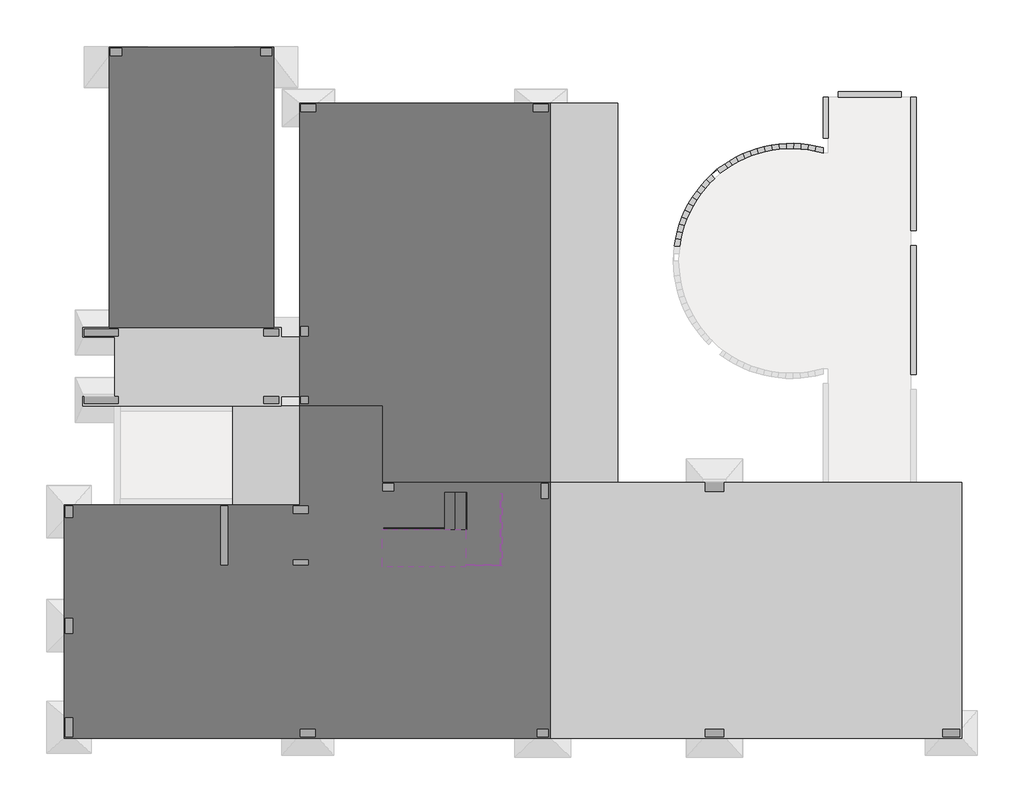
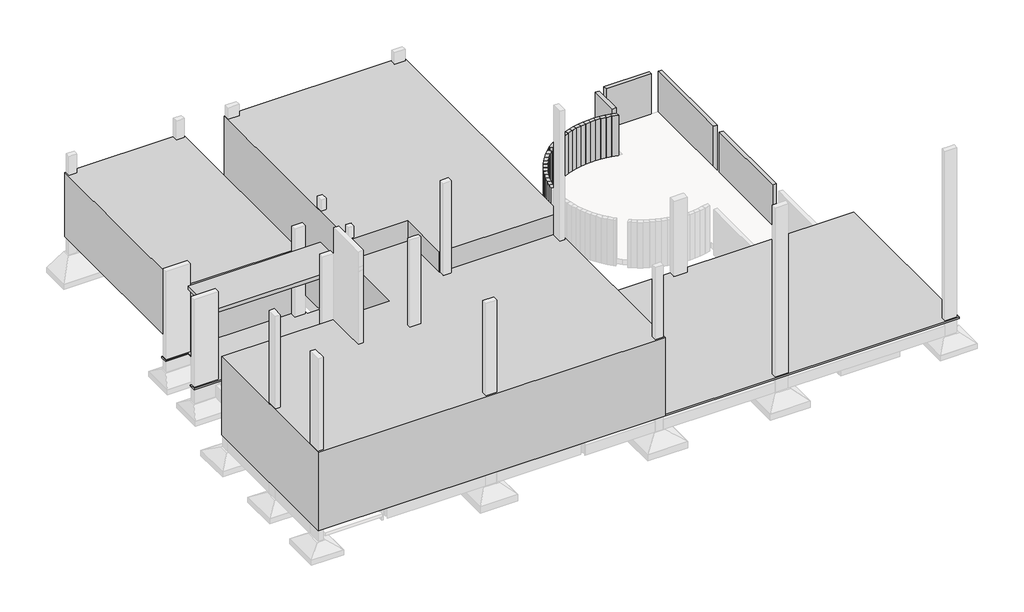
# One storey, part 4 of 4: 29 beams, 7 proxies, 6 railings, 2 stair flights, 1 slab.
"""IFC4 building model written with IfcOpenShell, lengths in millimetres."""

import ifcopenshell
import ifcopenshell.guid

model = None  # the IFC model being written
_history = None  # IfcOwnerHistory: only IFC2X3 demands one
_inside = {}  # id of a spatial element -> (the spatial element, [elements in it])
_under = {}  # id of a project, library or spatial element -> (it, [spatial elements below it])
_declared = {}  # id of a project -> (the project, [libraries it declares])
_typed = {}  # id of a type object -> (the type object, [elements of that type])
_made_of = {}  # id of a material, layer set ... -> (it, [elements and type objects made of it])


def new_model(schema):
    """Start an empty IFC model of exactly this schema.

    Asked for "IFC4X3", IfcOpenShell would pick the latest addendum, in which some entities
    have other attributes; the version numbers below select the first issue.
    IFC2X3 requires an IfcOwnerHistory on every rooted entity: one is made here for all.
    """
    global model, _history
    if schema == "IFC4X3":
        model = ifcopenshell.file(schema_version=(4, 3, 0, 0))
    else:
        model = ifcopenshell.file(schema=schema)
    _inside.clear()
    _under.clear()
    _declared.clear()
    _typed.clear()
    _made_of.clear()
    _history = None
    if model.schema == "IFC2X3":
        org = make("IfcOrganization", Name="unknown")
        user = make(
            "IfcPersonAndOrganization",
            ThePerson=make("IfcPerson", FamilyName="unknown"),
            TheOrganization=org,
        )
        app = make(
            "IfcApplication",
            ApplicationDeveloper=org,
            Version="unknown",
            ApplicationFullName="unknown",
            ApplicationIdentifier="unknown",
        )
        _history = make(
            "IfcOwnerHistory",
            OwningUser=user,
            OwningApplication=app,
            ChangeAction="ADDED",
            CreationDate=0,
        )
    return model


def make(cls, **values):
    """One entity of the class cls with the attributes given. An attribute that is None is left unset."""
    return model.create_entity(
        cls, **{name: value for name, value in values.items() if value is not None}
    )


def rooted(cls, **values):
    """An entity with a GlobalId (a new one), such as an element, a storey or a relation."""
    return make(cls, GlobalId=ifcopenshell.guid.new(), OwnerHistory=_history, **values)


def si_unit(unit_type, name, prefix=None):
    """IfcSIUnit, for example si_unit("LENGTHUNIT", "METRE", prefix="MILLI")."""
    return make("IfcSIUnit", UnitType=unit_type, Prefix=prefix, Name=name)


def assignment(units):
    """IfcUnitAssignment: the units of a project."""
    return None if units is None else make("IfcUnitAssignment", Units=units)


def point(xyz):
    """IfcCartesianPoint."""
    return None if xyz is None else make("IfcCartesianPoint", Coordinates=xyz)


def direction(xyz):
    """IfcDirection."""
    return None if xyz is None else make("IfcDirection", DirectionRatios=xyz)


def frame(location, z_axis=None, x_axis=None):
    """IfcAxis2Placement3D, a coordinate frame: its origin and axes. An axis left out is left unset."""
    return make(
        "IfcAxis2Placement3D",
        Location=point(location),
        Axis=direction(z_axis),
        RefDirection=direction(x_axis),
    )


def origin():
    """The frame at (0, 0, 0) with its axes left unset."""
    return frame((0.0, 0.0, 0.0))


def place(relative_to, where):
    """IfcLocalPlacement: puts the frame where relative to a parent placement (None: the world)."""
    return make(
        "IfcLocalPlacement", PlacementRelTo=relative_to, RelativePlacement=where
    )


def context(
    kind, dimensions, precision=None, world=None, true_north=None, identifier=None
):
    """IfcGeometricRepresentationContext, for example the 3D "Model" context."""
    return make(
        "IfcGeometricRepresentationContext",
        ContextIdentifier=identifier,
        ContextType=kind,
        CoordinateSpaceDimension=dimensions,
        Precision=precision,
        WorldCoordinateSystem=world,
        TrueNorth=true_north,
    )


def project(units=None, contexts=None):
    """IfcProject with its units and contexts."""
    return rooted(
        "IfcProject",
        Name="project",
        RepresentationContexts=contexts,
        UnitsInContext=assignment(units),
    )


def spatial(cls, under=None, at=None, **own):
    """A site, building, storey or space (cls), placed at a placement, below another one or the project."""
    s = rooted(cls, ObjectPlacement=at, **own)
    if under is not None:
        _under.setdefault(under.id(), (under, []))[1].append(s)
    return s


def polyline(points):
    """IfcPolyline through the points."""
    return make("IfcPolyline", Points=[point(p) for p in points])


def outline(outer, holes=None, kind="AREA"):
    """IfcArbitraryClosedProfileDef: a profile drawn as a closed curve; with holes, ...WithVoids."""
    if holes is None:
        return make("IfcArbitraryClosedProfileDef", ProfileType=kind, OuterCurve=outer)
    return make(
        "IfcArbitraryProfileDefWithVoids",
        ProfileType=kind,
        OuterCurve=outer,
        InnerCurves=holes,
    )


def extrude(swept, where, along, depth):
    """IfcExtrudedAreaSolid: the profile swept, set in the frame where, extruded along a direction by depth."""
    return make(
        "IfcExtrudedAreaSolid",
        SweptArea=swept,
        Position=where,
        ExtrudedDirection=direction(along),
        Depth=depth,
    )


def faces_of(points, faces, orient=None, outer=None):
    """IfcFace entities. A face is a list of loops; a loop is a list of indices into points, from 0.

    orient and outer hold one flag for each loop. By default every Orientation is true, the
    first loop of a face is its IfcFaceOuterBound and the others are IfcFaceBound.
    """
    made = []
    for i, loops in enumerate(faces):
        bounds = []
        for j, loop in enumerate(loops):
            is_outer = j == 0 if outer is None else outer[i][j]
            bounds.append(
                make(
                    "IfcFaceOuterBound" if is_outer else "IfcFaceBound",
                    Bound=make("IfcPolyLoop", Polygon=[points[k] for k in loop]),
                    Orientation=True if orient is None else orient[i][j],
                )
            )
        made.append(make("IfcFace", Bounds=bounds))
    return made


def faceted_brep(points, faces, orient=None, outer=None, voids=None):
    """IfcFacetedBrep: a solid bounded by flat faces; with voids (closed shells), ...WithVoids."""
    shared = [point(p) for p in points]
    hull = make("IfcClosedShell", CfsFaces=faces_of(shared, faces, orient, outer))
    if voids is None:
        return make("IfcFacetedBrep", Outer=hull)
    return make(
        "IfcFacetedBrepWithVoids",
        Outer=hull,
        Voids=[
            make(cls, CfsFaces=faces_of(shared, fs, o, b)) for cls, fs, o, b in voids
        ],
    )


def shape(context_of_items, identifier, shape_type, items):
    """IfcShapeRepresentation: the items that make up one representation, for example the "Body"."""
    return make(
        "IfcShapeRepresentation",
        ContextOfItems=context_of_items,
        RepresentationIdentifier=identifier,
        RepresentationType=shape_type,
        Items=items,
    )


def source(mapping_origin, context_of_items, identifier, shape_type, items):
    """IfcRepresentationMap: a shape defined once, which mapped items show again and again."""
    return make(
        "IfcRepresentationMap",
        MappingOrigin=mapping_origin,
        MappedRepresentation=shape(context_of_items, identifier, shape_type, items),
    )


def transform(
    local_origin,
    x_axis=None,
    y_axis=None,
    z_axis=None,
    scale=None,
    scale2=None,
    scale3=None,
    uniform=True,
):
    """IfcCartesianTransformationOperator3D, or its non-uniform kind. x_axis, y_axis, z_axis: its Axis1, 2, 3."""
    if uniform:
        return make(
            "IfcCartesianTransformationOperator3D",
            Axis1=direction(x_axis),
            Axis2=direction(y_axis),
            LocalOrigin=point(local_origin),
            Scale=scale,
            Axis3=direction(z_axis),
        )
    return make(
        "IfcCartesianTransformationOperator3DnonUniform",
        Axis1=direction(x_axis),
        Axis2=direction(y_axis),
        LocalOrigin=point(local_origin),
        Scale=scale,
        Axis3=direction(z_axis),
        Scale2=scale2,
        Scale3=scale3,
    )


def mapped(mapping_source, mapping_target):
    """IfcMappedItem: shows the shape of a source again, moved by a transform."""
    return make(
        "IfcMappedItem", MappingSource=mapping_source, MappingTarget=mapping_target
    )


def made_of(thing, what):
    """Note that an element or type object is made of a material, layer set ...; save() writes the relation."""
    if what is not None:
        _made_of.setdefault(what.id(), (what, []))[1].append(thing)
    return thing


def element(
    cls,
    number,
    at=None,
    inside=None,
    cuts=None,
    type_object=None,
    material=None,
    context=None,
    identifier="Body",
    shape_type=None,
    held_by="IfcProductDefinitionShape",
    body=None,
    shapes=None,
    **own,
):
    """One element of the class cls, such as IfcWall. Its Tag is "e" and its number.

    at: its placement. inside: the storey or other place that contains it. cuts: it is an
    opening in that element (IfcRelVoidsElement). A single representation is given by context,
    identifier, shape_type and body (its items); several are given by shapes. held_by: the class
    of the entity that holds the representations. save() writes the other relations.
    """
    e = rooted(cls, Tag="e%d" % number, ObjectPlacement=at, **own)
    if body is not None:
        shapes = [shape(context, identifier, shape_type, body)]
    if shapes is not None:
        e.Representation = make(held_by, Representations=shapes)
    if inside is not None:
        _inside.setdefault(inside.id(), (inside, []))[1].append(e)
    if cuts is not None:
        rooted(
            "IfcRelVoidsElement", RelatingBuildingElement=cuts, RelatedOpeningElement=e
        )
    if type_object is not None:
        _typed.setdefault(type_object.id(), (type_object, []))[1].append(e)
    return made_of(e, material)


def aggregate(whole, parts):
    """IfcRelAggregates: a whole, such as a stair, and the parts it consists of."""
    return rooted("IfcRelAggregates", RelatingObject=whole, RelatedObjects=parts)


def save(model, path):
    """Write the relations noted so far, then the file.

    IfcRelAggregates (storeys below a building ...), IfcRelContainedInSpatialStructure (elements
    in a storey), IfcRelDefinesByType, IfcRelAssociatesMaterial and IfcRelDeclares: one each for
    every whole, place, type object, material and project.
    """
    for whole, parts in _under.values():
        aggregate(whole, parts)
    for where, things in _inside.values():
        rooted(
            "IfcRelContainedInSpatialStructure",
            RelatedElements=things,
            RelatingStructure=where,
        )
    for kind, things in _typed.values():
        rooted("IfcRelDefinesByType", RelatedObjects=things, RelatingType=kind)
    for what, things in _made_of.values():
        rooted("IfcRelAssociatesMaterial", RelatedObjects=things, RelatingMaterial=what)
    for by, libraries in _declared.values():
        rooted("IfcRelDeclares", RelatingContext=by, RelatedDefinitions=libraries)
    model.write(path)


def railing_81dbcb3b(model_context):
    return source(origin(), model_context, "Body", "SweptSolid", [
        extrude(outline(polyline([(1832.4523952, 3702.0), (1832.4523952, 3594.0), (1856.4523952, 3594.0), (1856.4523952, 3702.0), (1866.9523952, 3702.0), (1866.9523952, 3700.0), (1858.4523952, 3700.0), (1858.4523952, 3592.0), (1830.4523952, 3592.0), (1830.4523952, 3700.0), (1821.9523952, 3700.0), (1821.9523952, 3702.0), (1832.4523952, 3702.0)])), frame((-12226.1487231, 0.0, 0.0), z_axis=(1.0, 0.0, 0.0), x_axis=(0.0, 1.0, 0.0)), (0.0, 0.0, 1.0), 1940.0),
    ])


def railing_0d959ca4(model_context):
    return source(origin(), model_context, "Body", "SweptSolid", [
        extrude(outline(polyline([(-4674.5702584, 2133.3602771), (-4674.5702584, 2121.3602771), (-6610.5702584, 2121.3602771), (-6610.5702584, 2133.3602771), (-4674.5702584, 2133.3602771)])), frame((0.0, 0.0, 4122.0679199), z_axis=(0.0, 0.0, 1.0), x_axis=(1.0, 0.0, 0.0)), (0.0, 0.0, 1.0), 1100.0),
    ])


def railing_24874f95(model_context):
    return source(origin(), model_context, "Body", "SweptSolid", [
        extrude(outline(polyline([(1832.4523952, 3702.0), (1832.4523952, 3594.0), (1856.4523952, 3594.0), (1856.4523952, 3702.0), (1866.9523952, 3702.0), (1866.9523952, 3700.0), (1858.4523952, 3700.0), (1858.4523952, 3592.0), (1830.4523952, 3592.0), (1830.4523952, 3700.0), (1821.9523952, 3700.0), (1821.9523952, 3702.0), (1832.4523952, 3702.0)])), frame((-12226.1487231, 0.0, 0.0), z_axis=(1.0, 0.0, 0.0), x_axis=(0.0, 1.0, 0.0)), (0.0, 0.0, 1.0), 925.0),
    ])


def railing_29f9e2f6(model_context):
    return source(origin(), model_context, "Body", "SweptSolid", [
        extrude(outline(polyline([(-4674.5702584, 2133.3602771), (-4674.5702584, 2121.3602771), (-5595.5702584, 2121.3602771), (-5595.5702584, 2133.3602771), (-4674.5702584, 2133.3602771)])), frame((0.0, 0.0, 4122.0679199), z_axis=(0.0, 0.0, 1.0), x_axis=(1.0, 0.0, 0.0)), (0.0, 0.0, 1.0), 1100.0),
    ])


def railing_c44cfcee(model_context):
    return source(origin(), model_context, "Body", "SweptSolid", [
        extrude(outline(polyline([(1672.2222222, -4460.281307), (500.0, -4460.281307), (1877.7777778, -2220.281307), (3050.0, -2220.281307), (1672.2222222, -4460.281307)])), frame((0.0, -5573.3699847, 0.0), z_axis=(0.0, 1.0, 0.0), x_axis=(0.0, 0.0, 1.0)), (0.0, 0.0, 1.0), 12.0),
    ])


model = new_model("IFC4")

# Units and contexts
model_context = context("Model", 3, world=origin())
ifc_project = project(units=[si_unit("LENGTHUNIT", "METRE", prefix="MILLI")], contexts=[model_context])

# Site, building, storey
site = spatial("IfcSite", under=ifc_project)
building = spatial("IfcBuilding", under=site)
storey = spatial("IfcBuildingStorey", under=building, Name="PAVIMENTO TÉRREO", Elevation=500.0)

# Beams
placement = place(None, origin())
element("IfcBeam", 1, ObjectType="TQS - Viga retangular : 14.0 x 180.0", at=placement, inside=storey, context=model_context, shape_type="SweptSolid", body=[
    extrude(outline(polyline([(9422.718693, 6109.4300153), (9422.718693, 5969.4300153), (7734.718693, 5969.4300153), (7734.718693, 6109.4300153), (9422.718693, 6109.4300153)])), frame((0.0, 0.0, -1450.0), z_axis=(0.0, 0.0, 1.0), x_axis=(1.0, 0.0, 0.0)), (0.0, 0.0, 1.0), 1800.0),
])
element("IfcBeam", 2, ObjectType="TQS - Viga retangular : 14.0 x 180.0", at=placement, inside=storey, context=model_context, shape_type="Brep", body=[
    faceted_brep([(3391.2860591, 2182.1270296, 350.0), (3359.6197005, 1984.821412, 350.0), (3498.5878389, 1967.228978, 350.0), (3528.8128087, 2155.5536418, 350.0), (3498.5878389, 1967.228978, -1250.0), (3498.5878389, 1967.228978, -1450.0), (3528.8128087, 2155.5536418, -1450.0), (3528.8128087, 2155.5536418, -1250.0), (3359.6197005, 1984.821412, -1450.0), (3391.2860591, 2182.1270296, -1450.0)], [[[0, 1, 2, 3]], [[3, 2, 4, 5, 6, 7]], [[6, 5, 8, 9]], [[1, 0, 9, 8]], [[1, 8, 5, 4, 2]], [[0, 3, 7, 6, 9]]]),
])
element("IfcBeam", 3, ObjectType="TQS - Viga retangular : 14.0 x 180.0", at=placement, inside=storey, context=model_context, shape_type="Brep", body=[
    faceted_brep([(3435.4949989, 2377.433408, 350.0), (3391.2860591, 2182.1270296, 350.0), (3528.8128087, 2155.5536418, 350.0), (3571.057344, 2342.1816685, 350.0), (3528.8128087, 2155.5536418, -1250.0), (3528.8128087, 2155.5536418, -1450.0), (3571.057344, 2342.1816685, -1450.0), (3571.057344, 2342.1816685, -1250.0), (3391.2860591, 2182.1270296, -1450.0), (3435.4949989, 2377.433408, -1450.0)], [[[0, 1, 2, 3]], [[3, 2, 4, 5, 6, 7]], [[6, 5, 8, 9]], [[1, 0, 9, 8]], [[1, 8, 5, 4, 2]], [[0, 3, 7, 6, 9]]]),
])
element("IfcBeam", 4, ObjectType="TQS - Viga retangular : 14.0 x 180.0", at=placement, inside=storey, context=model_context, shape_type="Brep", body=[
    faceted_brep([(3491.8466557, 2568.9190116, 350.0), (3435.4949989, 2377.433408, 350.0), (3571.057344, 2342.1816685, 350.0), (3624.8943566, 2525.1223914, 350.0), (3571.057344, 2342.1816685, -1250.0), (3571.057344, 2342.1816685, -1450.0), (3624.8943566, 2525.1223914, -1450.0), (3624.8943566, 2525.1223914, -1250.0), (3435.4949989, 2377.433408, -1450.0), (3491.8466557, 2568.9190116, -1450.0)], [[[0, 1, 2, 3]], [[3, 2, 4, 5, 6, 7]], [[6, 5, 8, 9]], [[1, 0, 9, 8]], [[1, 8, 5, 4, 2]], [[0, 3, 7, 6, 9]]]),
])
element("IfcBeam", 5, ObjectType="TQS - Viga retangular : 14.0 x 180.0", at=placement, inside=storey, context=model_context, shape_type="Brep", body=[
    faceted_brep([(3560.4750252, 2757.0390761, 350.0), (3491.8466557, 2568.9190116, 350.0), (3624.8943566, 2525.1223914, 350.0), (3690.4700641, 2704.8746778, 350.0), (3624.8943566, 2525.1223914, -1250.0), (3624.8943566, 2525.1223914, -1450.0), (3690.4700641, 2704.8746778, -1450.0), (3690.4700641, 2704.8746778, -1250.0), (3491.8466557, 2568.9190116, -1450.0), (3560.4750252, 2757.0390761, -1450.0)], [[[0, 1, 2, 3]], [[3, 2, 4, 5, 6, 7]], [[6, 5, 8, 9]], [[1, 0, 9, 8]], [[1, 8, 5, 4, 2]], [[0, 3, 7, 6, 9]]]),
])
element("IfcBeam", 6, ObjectType="TQS - Viga retangular : 14.0 x 180.0", at=placement, inside=storey, context=model_context, shape_type="Brep", body=[
    faceted_brep([(3640.6668309, 2939.8368394, 350.0), (3560.4750252, 2757.0390761, 350.0), (3690.4700641, 2704.8746778, 350.0), (3767.0835383, 2879.5156103, 350.0), (3690.4700641, 2704.8746778, -1250.0), (3690.4700641, 2704.8746778, -1450.0), (3767.0835383, 2879.5156103, -1450.0), (3767.0835383, 2879.5156103, -1250.0), (3560.4750252, 2757.0390761, -1450.0), (3640.6668309, 2939.8368394, -1450.0)], [[[0, 1, 2, 3]], [[3, 2, 4, 5, 6, 7]], [[6, 5, 8, 9]], [[1, 0, 9, 8]], [[1, 8, 5, 4, 2]], [[0, 3, 7, 6, 9]]]),
])
element("IfcBeam", 7, ObjectType="TQS - Viga retangular : 14.0 x 180.0", at=placement, inside=storey, context=model_context, shape_type="Brep", body=[
    faceted_brep([(3732.4184841, 3117.3686176, 350.0), (3640.6668309, 2939.8368394, 350.0), (3767.0835383, 2879.5156103, 350.0), (3854.7456543, 3049.1344759, 350.0), (3767.0835383, 2879.5156103, -1250.0), (3767.0835383, 2879.5156103, -1450.0), (3854.7456543, 3049.1344759, -1450.0), (3854.7456543, 3049.1344759, -1250.0), (3640.6668309, 2939.8368394, -1450.0), (3732.4184841, 3117.3686176, -1450.0)], [[[0, 1, 2, 3]], [[3, 2, 4, 5, 6, 7]], [[6, 5, 8, 9]], [[1, 0, 9, 8]], [[1, 8, 5, 4, 2]], [[0, 3, 7, 6, 9]]]),
])
element("IfcBeam", 8, ObjectType="TQS - Viga retangular : 14.0 x 180.0", at=placement, inside=storey, context=model_context, shape_type="Brep", body=[
    faceted_brep([(3835.4781404, 3289.0593829, 350.0), (3732.4184841, 3117.3686176, 350.0), (3854.7456543, 3049.1344759, 350.0), (3953.2211063, 3213.1882515, 350.0), (3854.7456543, 3049.1344759, -1250.0), (3854.7456543, 3049.1344759, -1450.0), (3953.2211063, 3213.1882515, -1450.0), (3953.2211063, 3213.1882515, -1250.0), (3732.4184841, 3117.3686176, -1450.0), (3835.4781404, 3289.0593829, -1450.0)], [[[0, 1, 2, 3]], [[3, 2, 4, 5, 6, 7]], [[6, 5, 8, 9]], [[1, 0, 9, 8]], [[1, 8, 5, 4, 2]], [[0, 3, 7, 6, 9]]]),
])
element("IfcBeam", 9, ObjectType="TQS - Viga retangular : 14.0 x 180.0", at=placement, inside=storey, context=model_context, shape_type="Brep", body=[
    faceted_brep([(3949.2418511, 3453.852677, 350.0), (3835.4781404, 3289.0593829, 350.0), (3953.2211063, 3213.1882515, 350.0), (4061.9244879, 3370.6513671, 350.0), (3953.2211063, 3213.1882515, -1250.0), (3953.2211063, 3213.1882515, -1450.0), (4061.9244879, 3370.6513671, -1450.0), (4061.9244879, 3370.6513671, -1250.0), (3835.4781404, 3289.0593829, -1450.0), (3949.2418511, 3453.852677, -1450.0)], [[[0, 1, 2, 3]], [[3, 2, 4, 5, 6, 7]], [[6, 5, 8, 9]], [[1, 0, 9, 8]], [[1, 8, 5, 4, 2]], [[0, 3, 7, 6, 9]]]),
])
element("IfcBeam", 10, ObjectType="TQS - Viga retangular : 14.0 x 180.0", at=placement, inside=storey, context=model_context, shape_type="Brep", body=[
    faceted_brep([(4073.2495799, 3611.0821108, 350.0), (3949.2418511, 3453.852677, 350.0), (4061.9244879, 3370.6513671, 350.0), (4180.416223, 3520.8870709, 350.0), (4061.9244879, 3370.6513671, -1250.0), (4061.9244879, 3370.6513671, -1450.0), (4180.416223, 3520.8870709, -1450.0), (4180.416223, 3520.8870709, -1250.0), (3949.2418511, 3453.852677, -1450.0), (4073.2495799, 3611.0821108, -1450.0)], [[[0, 1, 2, 3]], [[3, 2, 4, 5, 6, 7]], [[6, 5, 8, 9]], [[1, 0, 9, 8]], [[1, 8, 5, 4, 2]], [[0, 3, 7, 6, 9]]]),
])
element("IfcBeam", 11, ObjectType="TQS - Viga retangular : 14.0 x 180.0", at=placement, inside=storey, context=model_context, shape_type="Brep", body=[
    faceted_brep([(4206.9998658, 3760.1118816, 350.0), (4073.2495799, 3611.0821108, 350.0), (4180.416223, 3520.8870709, 350.0), (4308.2171619, 3663.2878479, 350.0), (4180.416223, 3520.8870709, -1250.0), (4180.416223, 3520.8870709, -1450.0), (4308.2171619, 3663.2878479, -1450.0), (4308.2171619, 3663.2878479, -1250.0), (4073.2495799, 3611.0821108, -1450.0), (4206.9998658, 3760.1118816, -1450.0)], [[[0, 1, 2, 3]], [[3, 2, 4, 5, 6, 7]], [[6, 5, 8, 9]], [[1, 0, 9, 8]], [[1, 8, 5, 4, 2]], [[0, 3, 7, 6, 9]]]),
])
element("IfcBeam", 12, ObjectType="TQS - Viga retangular : 14.0 x 180.0", at=placement, inside=storey, context=model_context, shape_type="Brep", body=[
    faceted_brep([(4505.0858129, 4030.990239, 350.0), (4495.3853819, 4043.0011294, 350.0), (4357.8172159, 3908.0548411, 350.0), (4500.8039544, 4027.7001668, 350.0), (4495.3853819, 4043.0011294, -1450.0), (4505.0858129, 4030.990239, -1450.0), (4500.8039544, 4027.7001668, -1450.0), (4357.8172159, 3908.0548411, -1450.0)], [[[0, 1, 2, 3]], [[4, 5, 6, 7]], [[1, 4, 7, 2]], [[4, 1, 0, 5]], [[3, 6, 5, 0]], [[6, 3, 2, 7]]]),
    faceted_brep([(4433.7325967, 3786.411115, 350.0), (4308.2171619, 3663.2878479, 350.0), (4308.2171619, 3663.2878479, -1250.0), (4308.2171619, 3663.2878479, -1450.0), (4433.7325967, 3786.411115, -1450.0), (4433.7325967, 3786.411115, -1250.0), (4346.9865149, 3897.4305598, 350.0), (4346.9865149, 3897.4305598, -1450.0), (4206.9998658, 3760.1118816, 350.0), (4206.9998658, 3760.1118816, -1450.0)], [[[0, 1, 2, 3, 4, 5]], [[6, 0, 5, 4, 7]], [[8, 9, 3, 2, 1]], [[1, 0, 6, 8]], [[4, 3, 9, 7]], [[6, 7, 9, 8]]]),
])
element("IfcBeam", 13, ObjectType="TQS - Viga retangular : 14.0 x 180.0", at=placement, inside=storey, context=model_context, shape_type="Brep", body=[
    faceted_brep([(4707.2476524, 4182.7114576, 350.0), (4495.3853819, 4043.0011294, 350.0), (4505.0858129, 4030.990239, 350.0), (4583.7591724, 3933.5783713, 350.0), (4784.4362281, 4065.9127281, 350.0), (4583.7591724, 3933.5783713, -1450.0), (4742.6545701, 4038.3602567, -1450.0), (4784.4362281, 4065.9127281, -1450.0), (4784.4362281, 4065.9127281, -1250.0), (4495.3853819, 4043.0011294, -1450.0), (4707.2476524, 4182.7114576, -1450.0), (4505.0858129, 4030.990239, -1450.0)], [[[0, 1, 2, 3, 4]], [[4, 3, 5, 6, 7, 8]], [[9, 10, 7, 6, 5, 11]], [[1, 0, 10, 9]], [[1, 9, 11, 5, 3, 2]], [[0, 4, 8, 7, 10]]]),
])
element("IfcBeam", 14, ObjectType="TQS - Viga retangular : 14.0 x 180.0", at=placement, inside=storey, context=model_context, shape_type="Brep", body=[
    faceted_brep([(4828.0654459, 4262.728967, 350.0), (4707.2476524, 4182.7114576, 350.0), (4784.4362281, 4065.9127281, 350.0), (4901.6570883, 4143.547992, 350.0), (4784.4362281, 4065.9127281, -1250.0), (4784.4362281, 4065.9127281, -1450.0), (4901.6570883, 4143.547992, -1450.0), (4901.6570883, 4143.547992, -1250.0), (4707.2476524, 4182.7114576, -1450.0), (4828.0654459, 4262.728967, -1450.0)], [[[0, 1, 2, 3]], [[3, 2, 4, 5, 6, 7]], [[6, 5, 8, 9]], [[1, 0, 9, 8]], [[1, 8, 5, 4, 2]], [[0, 3, 7, 6, 9]]]),
])
element("IfcBeam", 15, ObjectType="TQS - Viga retangular : 14.0 x 180.0", at=placement, inside=storey, context=model_context, shape_type="Brep", body=[
    faceted_brep([(5001.7073563, 4362.4661134, 350.0), (4828.0654459, 4262.728967, 350.0), (4901.6570883, 4143.547992, 350.0), (5067.5752245, 4238.8487257, 350.0), (4901.6570883, 4143.547992, -1250.0), (4901.6570883, 4143.547992, -1450.0), (5067.5752245, 4238.8487257, -1450.0), (5067.5752245, 4238.8487257, -1250.0), (4828.0654459, 4262.728967, -1450.0), (5001.7073563, 4362.4661134, -1450.0)], [[[0, 1, 2, 3]], [[3, 2, 4, 5, 6, 7]], [[6, 5, 8, 9]], [[1, 0, 9, 8]], [[1, 8, 5, 4, 2]], [[0, 3, 7, 6, 9]]]),
])
element("IfcBeam", 16, ObjectType="TQS - Viga retangular : 14.0 x 180.0", at=placement, inside=storey, context=model_context, shape_type="Brep", body=[
    faceted_brep([(5181.3373377, 4450.9651597, 350.0), (5001.7073563, 4362.4661134, 350.0), (5067.5752245, 4238.8487257, 350.0), (5239.2150761, 4323.4112417, 350.0), (5067.5752245, 4238.8487257, -1250.0), (5067.5752245, 4238.8487257, -1450.0), (5239.2150761, 4323.4112417, -1450.0), (5239.2150761, 4323.4112417, -1250.0), (5001.7073563, 4362.4661134, -1450.0), (5181.3373377, 4450.9651597, -1450.0)], [[[0, 1, 2, 3]], [[3, 2, 4, 5, 6, 7]], [[6, 5, 8, 9]], [[1, 0, 9, 8]], [[1, 8, 5, 4, 2]], [[0, 3, 7, 6, 9]]]),
])
element("IfcBeam", 17, ObjectType="TQS - Viga retangular : 14.0 x 180.0", at=placement, inside=storey, context=model_context, shape_type="Brep", body=[
    faceted_brep([(5366.2290044, 4527.8682345, 350.0), (5181.3373377, 4450.9651597, 350.0), (5239.2150761, 4323.4112417, 350.0), (5415.8825678, 4396.8935871, 350.0), (5239.2150761, 4323.4112417, -1250.0), (5239.2150761, 4323.4112417, -1450.0), (5415.8825678, 4396.8935871, -1450.0), (5415.8825678, 4396.8935871, -1250.0), (5181.3373377, 4450.9651597, -1450.0), (5366.2290044, 4527.8682345, -1450.0)], [[[0, 1, 2, 3]], [[3, 2, 4, 5, 6, 7]], [[6, 5, 8, 9]], [[1, 0, 9, 8]], [[1, 8, 5, 4, 2]], [[0, 3, 7, 6, 9]]]),
])
element("IfcBeam", 18, ObjectType="TQS - Viga retangular : 14.0 x 180.0", at=placement, inside=storey, context=model_context, shape_type="Brep", body=[
    faceted_brep([(5555.634694, 4592.8643582, 350.0), (5366.2290044, 4527.8682345, 350.0), (5415.8825678, 4396.8935871, 350.0), (5596.8632938, 4458.9986151, 350.0), (5415.8825678, 4396.8935871, -1250.0), (5415.8825678, 4396.8935871, -1450.0), (5596.8632938, 4458.9986151, -1450.0), (5596.8632938, 4458.9986151, -1250.0), (5366.2290044, 4527.8682345, -1450.0), (5555.634694, 4592.8643582, -1450.0)], [[[0, 1, 2, 3]], [[3, 2, 4, 5, 6, 7]], [[6, 5, 8, 9]], [[1, 0, 9, 8]], [[1, 8, 5, 4, 2]], [[0, 3, 7, 6, 9]]]),
])
element("IfcBeam", 19, ObjectType="TQS - Viga retangular : 14.0 x 180.0", at=placement, inside=storey, context=model_context, shape_type="Brep", body=[
    faceted_brep([(5748.78849, 4645.6907002, 350.0), (5555.634694, 4592.8643582, 350.0), (5596.8632938, 4458.9986151, 350.0), (5781.4254065, 4509.475186, 350.0), (5596.8632938, 4458.9986151, -1250.0), (5596.8632938, 4458.9986151, -1450.0), (5781.4254065, 4509.475186, -1450.0), (5781.4254065, 4509.475186, -1250.0), (5555.634694, 4592.8643582, -1450.0), (5748.78849, 4645.6907002, -1450.0)], [[[0, 1, 2, 3]], [[3, 2, 4, 5, 6, 7]], [[6, 5, 8, 9]], [[1, 0, 9, 8]], [[1, 8, 5, 4, 2]], [[0, 3, 7, 6, 9]]]),
])
element("IfcBeam", 20, ObjectType="TQS - Viga retangular : 14.0 x 180.0", at=placement, inside=storey, context=model_context, shape_type="Brep", body=[
    faceted_brep([(5944.9093194, 4686.133642, 350.0), (5748.78849, 4645.6907002, 350.0), (5781.4254065, 4509.475186, 350.0), (5968.8225759, 4548.1191834, 350.0), (5781.4254065, 4509.475186, -1250.0), (5781.4254065, 4509.475186, -1450.0), (5968.8225759, 4548.1191834, -1450.0), (5968.8225759, 4548.1191834, -1250.0), (5748.78849, 4645.6907002, -1450.0), (5944.9093194, 4686.133642, -1450.0)], [[[0, 1, 2, 3]], [[3, 2, 4, 5, 6, 7]], [[6, 5, 8, 9]], [[1, 0, 9, 8]], [[1, 8, 5, 4, 2]], [[0, 3, 7, 6, 9]]]),
])
element("IfcBeam", 21, ObjectType="TQS - Viga retangular : 14.0 x 180.0", at=placement, inside=storey, context=model_context, shape_type="Brep", body=[
    faceted_brep([(6143.2041112, 4714.029641, 350.0), (5944.9093194, 4686.133642, 350.0), (5968.8225759, 4548.1191834, 350.0), (6158.2970076, 4574.7743392, 350.0), (5968.8225759, 4548.1191834, -1250.0), (5968.8225759, 4548.1191834, -1450.0), (6158.2970076, 4574.7743392, -1450.0), (6158.2970076, 4574.7743392, -1250.0), (5944.9093194, 4686.133642, -1450.0), (6143.2041112, 4714.029641, -1450.0)], [[[0, 1, 2, 3]], [[3, 2, 4, 5, 6, 7]], [[6, 5, 8, 9]], [[1, 0, 9, 8]], [[1, 8, 5, 4, 2]], [[0, 3, 7, 6, 9]]]),
])
element("IfcBeam", 22, ObjectType="TQS - Viga retangular : 14.0 x 180.0", at=placement, inside=storey, context=model_context, shape_type="Brep", body=[
    faceted_brep([(6342.8710035, 4729.2658917, 350.0), (6143.2041112, 4714.029641, 350.0), (6158.2970076, 4574.7743392, 350.0), (6349.0825072, 4589.3328655, 350.0), (6158.2970076, 4574.7743392, -1250.0), (6158.2970076, 4574.7743392, -1450.0), (6349.0825072, 4589.3328655, -1450.0), (6349.0825072, 4589.3328655, -1250.0), (6143.2041112, 4714.029641, -1450.0), (6342.8710035, 4729.2658917, -1450.0)], [[[0, 1, 2, 3]], [[3, 2, 4, 5, 6, 7]], [[6, 5, 8, 9]], [[1, 0, 9, 8]], [[1, 8, 5, 4, 2]], [[0, 3, 7, 6, 9]]]),
])
element("IfcBeam", 23, ObjectType="TQS - Viga retangular : 14.0 x 180.0", at=placement, inside=storey, context=model_context, shape_type="Brep", body=[
    faceted_brep([(6543.1025857, 4731.7807819, 350.0), (6342.8710035, 4729.2658917, 350.0), (6349.0825072, 4589.3328655, 350.0), (6540.4075788, 4591.7358908, 350.0), (6349.0825072, 4589.3328655, -1250.0), (6349.0825072, 4589.3328655, -1450.0), (6540.4075788, 4591.7358908, -1450.0), (6540.4075788, 4591.7358908, -1250.0), (6342.8710035, 4729.2658917, -1450.0), (6543.1025857, 4731.7807819, -1450.0)], [[[0, 1, 2, 3]], [[3, 2, 4, 5, 6, 7]], [[6, 5, 8, 9]], [[1, 0, 9, 8]], [[1, 8, 5, 4, 2]], [[0, 3, 7, 6, 9]]]),
])
element("IfcBeam", 24, ObjectType="TQS - Viga retangular : 14.0 x 180.0", at=placement, inside=storey, context=model_context, shape_type="Brep", body=[
    faceted_brep([(6743.0891637, 4721.5641421, 350.0), (6543.1025857, 4731.7807819, 350.0), (6540.4075788, 4591.7358908, 350.0), (6731.4985443, 4581.9736977, 350.0), (6540.4075788, 4591.7358908, -1250.0), (6540.4075788, 4591.7358908, -1450.0), (6731.4985443, 4581.9736977, -1450.0), (6731.4985443, 4581.9736977, -1250.0), (6543.1025857, 4731.7807819, -1450.0), (6743.0891637, 4721.5641421, -1450.0)], [[[0, 1, 2, 3]], [[3, 2, 4, 5, 6, 7]], [[6, 5, 8, 9]], [[1, 0, 9, 8]], [[1, 8, 5, 4, 2]], [[0, 3, 7, 6, 9]]]),
])
element("IfcBeam", 25, ObjectType="TQS - Viga retangular : 14.0 x 180.0", at=placement, inside=storey, context=model_context, shape_type="Brep", body=[
    faceted_brep([(6942.0220345, 4698.657286, 350.0), (6743.0891637, 4721.5641421, 350.0), (6731.4985443, 4581.9736977, 350.0), (6921.5826725, 4560.0857626, 350.0), (6731.4985443, 4581.9736977, -1250.0), (6731.4985443, 4581.9736977, -1450.0), (6921.5826725, 4560.0857626, -1450.0), (6921.5826725, 4560.0857626, -1250.0), (6743.0891637, 4721.5641421, -1450.0), (6942.0220345, 4698.657286, -1450.0)], [[[0, 1, 2, 3]], [[3, 2, 4, 5, 6, 7]], [[6, 5, 8, 9]], [[1, 0, 9, 8]], [[1, 8, 5, 4, 2]], [[0, 3, 7, 6, 9]]]),
])
element("IfcBeam", 26, ObjectType="TQS - Viga retangular : 14.0 x 180.0", at=placement, inside=storey, context=model_context, shape_type="Brep", body=[
    faceted_brep([(7139.0967556, 4663.1528442, 350.0), (6942.0220345, 4698.657286, 350.0), (6921.5826725, 4560.0857626, 350.0), (7109.8912551, 4526.1606043, 350.0), (6921.5826725, 4560.0857626, -1250.0), (6921.5826725, 4560.0857626, -1450.0), (7109.8912551, 4526.1606043, -1450.0), (7109.8912551, 4526.1606043, -1250.0), (6942.0220345, 4698.657286, -1450.0), (7139.0967556, 4663.1528442, -1450.0)], [[[0, 1, 2, 3]], [[3, 2, 4, 5, 6, 7]], [[6, 5, 8, 9]], [[1, 0, 9, 8]], [[1, 8, 5, 4, 2]], [[0, 3, 7, 6, 9]]]),
])
element("IfcBeam", 27, ObjectType="TQS - Viga retangular : 14.0 x 180.0", at=placement, inside=storey, context=model_context, shape_type="Brep", body=[
    faceted_brep([(7109.8912551, 4526.1606043, 350.0), (7334.7218272, 4470.7003679, 350.0), (7334.7218272, 4614.8968948, 350.0), (7139.0967556, 4663.1528442, 350.0), (7109.8912551, 4526.1606043, -1250.0), (7109.8912551, 4526.1606043, -1450.0), (7334.7218272, 4470.7003679, -1450.0), (7334.7218272, 4470.7003679, -1250.0), (7139.0967556, 4663.1528442, -1450.0), (7334.7218272, 4614.8968948, -1450.0)], [[[0, 1, 2, 3]], [[1, 0, 4, 5, 6, 7]], [[6, 5, 8, 9]], [[3, 2, 9, 8]], [[2, 1, 7, 6, 9]], [[3, 8, 5, 4, 0]]]),
])
element("IfcBeam", 28, ObjectType="TQS - Viga retangular : 14.0 x 180.0", at=placement, inside=storey, context=model_context, shape_type="Brep", body=[
    faceted_brep([(7334.7218272, 5969.4300153, 350.0), (7334.7218272, 4870.7003679, 350.0), (7474.7218272, 4870.7003679, 350.0), (7474.7218272, 5969.4300153, 350.0), (7474.7218272, 4870.7003679, -1250.0), (7474.7218272, 4870.7003679, -1450.0), (7474.7218272, 5969.4300153, -1450.0), (7474.7218272, 5969.4300153, -1250.0), (7334.7218272, 4870.7003679, -1450.0), (7334.7218272, 5969.4300153, -1450.0)], [[[0, 1, 2, 3]], [[3, 2, 4, 5, 6, 7]], [[6, 5, 8, 9]], [[1, 0, 9, 8]], [[0, 3, 7, 6, 9]], [[1, 8, 5, 4, 2]]]),
])
element("IfcBeam", 29, ObjectType="TQS - Viga retangular : 14.0 x 180.0", at=placement, inside=storey, context=model_context, shape_type="Brep", body=[
    faceted_brep([(9822.718693, 5969.4300153, 350.0), (9682.718693, 5969.4300153, 350.0), (9682.718693, 2394.0144504, 350.0), (9822.718693, 2394.0144504, 350.0), (9822.718693, 5969.4300153, -1450.0), (9822.718693, 2394.0144504, -1450.0), (9682.718693, 5969.4300153, -1450.0), (9682.718693, 2394.0144504, -1450.0), (9682.718693, 5969.4300153, -1250.0)], [[[0, 1, 2, 3]], [[4, 0, 3, 5]], [[6, 4, 5, 7]], [[1, 8, 6, 7, 2]], [[3, 2, 7, 5]], [[1, 0, 4, 6, 8]]]),
    faceted_brep([(9822.718693, -1451.4011146, 350.0), (9682.718693, -1451.4011146, 350.0), (9682.718693, -1451.4011146, -1450.0), (9822.718693, -1451.4011146, -1450.0), (9682.718693, 1994.0144504, 350.0), (9822.718693, 1994.0144504, 350.0), (9822.718693, 1994.0144504, -1450.0), (9682.718693, 1994.0144504, -1450.0)], [[[0, 1, 2, 3]], [[4, 5, 6, 7]], [[1, 0, 5, 4]], [[0, 3, 6, 5]], [[3, 2, 7, 6]], [[2, 1, 4, 7]]]),
])

# Proxies
element("IfcBuildingElementProxy", 30, Name="GARAGEM : GARAGEM", ObjectType="GARAGEM : GARAGEM", at=placement, inside=storey, context=model_context, shape_type="SweptSolid", body=[
    extrude(outline(polyline([(-7360.281307, 7304.4300153), (-7360.281307, -195.5699847), (-11760.281307, -195.5699847), (-11760.281307, 7304.4300153), (-7360.281307, 7304.4300153)])), frame((0.0, 0.0, 500.0), z_axis=(0.0, 0.0, 1.0), x_axis=(1.0, 0.0, 0.0)), (0.0, 0.0, 1.0), 2550.0),
])
element("IfcBuildingElementProxy", 31, Name="PERGOLADO SALAS : PERGOLADO SALAS", ObjectType="PERGOLADO SALAS : PERGOLADO SALAS", at=placement, inside=storey, context=model_context, shape_type="SweptSolid", body=[
    extrude(outline(polyline([(1839.718693, 5804.4300153), (1839.718693, -4345.5699847), (39.718693, -4345.5699847), (39.718693, 5804.4300153), (1839.718693, 5804.4300153)])), frame((0.0, 0.0, 500.0), z_axis=(0.0, 0.0, 1.0), x_axis=(1.0, 0.0, 0.0)), (0.0, 0.0, 1.0), 50.0),
])
element("IfcBuildingElementProxy", 32, Name="VARANDA GOURMET : VARANDA GOURMET", ObjectType="VARANDA GOURMET : VARANDA GOURMET", at=placement, inside=storey, context=model_context, shape_type="SweptSolid", body=[
    extrude(outline(polyline([(11039.718693, -4345.5699847), (11039.718693, -11195.5699847), (39.718693, -11195.5699847), (39.718693, -4345.5699847), (11039.718693, -4345.5699847)])), frame((0.0, 0.0, 500.0), z_axis=(0.0, 0.0, 1.0), x_axis=(1.0, 0.0, 0.0)), (0.0, 0.0, 1.0), 50.0),
])
element("IfcBuildingElementProxy", 33, Name="PÓRTICO ENTRADA : PÓRTICO ENTRADA", ObjectType="PÓRTICO ENTRADA : PÓRTICO ENTRADA", at=placement, inside=storey, context=model_context, shape_type="SweptSolid", body=[
    extrude(outline(polyline([(-7160.281307, -445.5699847), (-6660.281307, -445.5699847), (-6660.281307, -2045.5699847), (-7160.281307, -2045.5699847), (-7160.281307, -2295.5699847), (-12460.281307, -2295.5699847), (-12460.281307, -2045.5699847), (-11610.281307, -2045.5699847), (-11610.281307, -445.5699847), (-12460.281307, -445.5699847), (-12460.281307, -195.5699847), (-7160.281307, -195.5699847), (-7160.281307, -445.5699847)])), frame((0.0, 0.0, 500.0), z_axis=(0.0, 0.0, 1.0), x_axis=(1.0, 0.0, 0.0)), (0.0, 0.0, 1.0), 50.0),
    extrude(outline(polyline([(-6660.281307, -445.5699847), (-6660.281307, -2045.5699847), (-11610.281307, -2045.5699847), (-11610.281307, -445.5699847), (-6660.281307, -445.5699847)])), frame((0.0, 0.0, 3050.0), z_axis=(0.0, 0.0, 1.0), x_axis=(1.0, 0.0, 0.0)), (0.0, 0.0, 1.0), 150.0),
])
element("IfcBuildingElementProxy", 34, Name="SALAS : SALAS", ObjectType="SALAS : SALAS", at=placement, inside=storey, context=model_context, shape_type="SweptSolid", body=[
    extrude(outline(polyline([(39.718693, 5804.4300153), (39.718693, -4345.5699847), (-4460.281307, -4345.5699847), (-4460.281307, -2295.5699847), (-6660.281307, -2295.5699847), (-6660.281307, 5804.4300153), (39.718693, 5804.4300153)])), frame((0.0, 0.0, 500.0), z_axis=(0.0, 0.0, 1.0), x_axis=(1.0, 0.0, 0.0)), (0.0, 0.0, 1.0), 3900.0),
])
element("IfcBuildingElementProxy", 35, Name="PROJEÇÃO : PROJEÇÃO", ObjectType="PROJEÇÃO : PROJEÇÃO", at=placement, inside=storey, context=model_context, shape_type="SweptSolid", body=[
    extrude(outline(polyline([(-6660.281307, -2295.5699847), (-6660.281307, -4945.5699847), (-8460.281307, -4945.5699847), (-8460.281307, -2295.5699847), (-6660.281307, -2295.5699847)])), frame((0.0, 0.0, 500.0), z_axis=(0.0, 0.0, 1.0), x_axis=(1.0, 0.0, 0.0)), (0.0, 0.0, 1.0), 50.0),
])
element("IfcBuildingElementProxy", 36, Name="COZINHA E LAVANDERIA : COZINHA E LAVANDERIA", ObjectType="COZINHA E LAVANDERIA : COZINHA E LAVANDERIA", at=placement, inside=storey, context=model_context, shape_type="SweptSolid", body=[
    extrude(outline(polyline([(-4460.281307, -4345.5699847), (39.718693, -4345.5699847), (39.718693, -11195.5699847), (-12960.281307, -11195.5699847), (-12960.281307, -4945.5699847), (-6660.281307, -4945.5699847), (-6660.281307, -2295.5699847), (-4460.281307, -2295.5699847), (-4460.281307, -4345.5699847)])), frame((0.0, 0.0, 500.0), z_axis=(0.0, 0.0, 1.0), x_axis=(1.0, 0.0, 0.0)), (0.0, 0.0, 1.0), 3100.0),
])

# Railings
railing_shape = railing_81dbcb3b(model_context)
element("IfcRailing", 37, ObjectType="ML_Perfil U de embutir3 : ML_Perfil U de embutir", at=placement, inside=storey, context=model_context, shape_type="MappedRepresentation", body=[
    mapped(railing_shape, transform((-3117.2337022, -16861.5187078, -1650.0), x_axis=(0.0, -1.0, 0.0), y_axis=(1.0, 0.0, 0.0), z_axis=(0.0, 0.0, 1.0))),
])
railing_2_shape = railing_0d959ca4(model_context)
element("IfcRailing", 38, ObjectType="ML_Painéis3 : ML_Painéis", at=placement, inside=storey, context=model_context, shape_type="MappedRepresentation", body=[
    mapped(railing_2_shape, transform((-3400.141584, -11247.9402431, -2172.0679199), x_axis=(0.0, -1.0, 0.0), y_axis=(1.0, 0.0, 0.0), z_axis=(0.0, 0.0, 1.0))),
])
railing_3_shape = railing_24874f95(model_context)
element("IfcRailing", 39, ObjectType="ML_Perfil U de embutir4 : ML_Perfil U de embutir", at=placement, inside=storey, context=model_context, shape_type="MappedRepresentation", body=[
    mapped(railing_3_shape, transform((10005.8674161, -8397.3223799, -1650.0), x_axis=(1.0, 0.0, 0.0), y_axis=(0.0, 1.0, 0.0), z_axis=(0.0, 0.0, 1.0))),
])
railing_4_shape = railing_29f9e2f6(model_context)
element("IfcRailing", 40, ObjectType="ML_Painéis4 : ML_Painéis", at=placement, inside=storey, context=model_context, shape_type="MappedRepresentation", body=[
    mapped(railing_4_shape, transform((3377.2889515, -8680.2302618, -2172.0679199), x_axis=(1.0, 0.0, 0.0), y_axis=(0.0, 1.0, 0.0), z_axis=(0.0, 0.0, 1.0))),
])
railing_5_shape = railing_c44cfcee(model_context)
element("IfcRailing", 41, ObjectType="ML_Guarda_corpo lance : ML_Guarda_corpo lance", at=placement, inside=storey, context=model_context, shape_type="MappedRepresentation", body=[
    mapped(railing_5_shape, transform((0.0, 0.0, 0.0), x_axis=(1.0, 0.0, 0.0), y_axis=(0.0, 1.0, 0.0), z_axis=(0.0, 0.0, 1.0))),
])
element("IfcRailing", 42, ObjectType="ML_Guarda_corpo lance1 : ML_Guarda_corpo lance", at=placement, inside=storey, context=model_context, shape_type="MappedRepresentation", body=[
    mapped(railing_5_shape, transform((0.0, 0.0, 0.0), x_axis=(1.0, 0.0, 0.0), y_axis=(0.0, 1.0, 0.0), z_axis=(0.0, 0.0, 1.0))),
])

# Slab
element("IfcSlab", 43, ObjectType="Espessura de 300 mm", at=placement, inside=storey, context=model_context, shape_type="SolidModel", body=[
    faceted_brep([(-2220.281307, -4605.3699847, 2030.0), (-2220.281307, -5605.3699847, 2030.0), (-2220.281307, -6605.3699847, 2030.0), (-2018.8487302, -6605.3699847, 2030.0), (-1220.281307, -6605.3699847, 2030.0), (-1220.281307, -4605.3699847, 2030.0), (-2141.7138837, -4605.3699847, 2030.0), (-2220.281307, -4605.3699847, 1857.7777778), (-2220.281307, -4605.3699847, 1681.6747992), (-2220.281307, -5605.3699847, 1681.6747992), (-2220.281307, -5605.3699847, 1853.8970214), (-2220.281307, -6605.3699847, 1853.8970214), (-2018.8487302, -6605.3699847, 1730.0), (-1220.281307, -6605.3699847, 1730.0), (-1220.281307, -4605.3699847, 1730.0), (-2141.7138837, -4605.3699847, 1730.0), (-2018.8487302, -5605.3699847, 1730.0), (-2141.7138837, -5605.3699847, 1730.0), (-2141.7138837, -5605.3699847, 1805.5718206)], [[[0, 1, 2, 3, 4, 5, 6]], [[1, 0, 7, 8, 9, 10]], [[2, 1, 10, 11]], [[2, 11, 12, 13, 4, 3]], [[5, 4, 13, 14]], [[8, 7, 0, 6, 5, 14, 15]], [[16, 17, 15, 14, 13, 12]], [[17, 16, 18]], [[15, 17, 9, 8]], [[17, 18, 10, 9]], [[16, 12, 11, 10, 18]]]),
    extrude(outline(polyline([(-2220.281307, -4605.3699847), (-1220.281307, -4605.3699847), (-1220.281307, -6605.3699847), (-2220.281307, -6605.3699847), (-2220.281307, -5605.3699847), (-2220.281307, -4605.3699847)])), frame((0.0, 0.0, 2030.0), z_axis=(0.0, 0.0, 1.0), x_axis=(1.0, 0.0, 0.0)), (0.0, 0.0, 1.0), 20.0),
])

# Stair flights
element("IfcStairFlight", 44, ObjectType="Profundidade de 150 mm - SEM BOCEL", at=placement, inside=storey, context=model_context, shape_type="SolidModel", body=[
    faceted_brep([(-4180.281307, -4605.3699847, 652.2222222), (-4460.281307, -4605.3699847, 652.2222222), (-4460.281307, -5605.3699847, 652.2222222), (-4180.281307, -5605.3699847, 652.2222222), (-4180.281307, -4605.3699847, 500.0), (-4460.281307, -4605.3699847, 500.0), (-4460.281307, -5605.3699847, 500.0), (-4180.281307, -5605.3699847, 500.0), (-3900.281307, -4605.3699847, 824.4444444), (-4180.281307, -4605.3699847, 824.4444444), (-4180.281307, -5605.3699847, 824.4444444), (-3900.281307, -5605.3699847, 824.4444444), (-3900.281307, -4605.3699847, 648.3414658), (-4141.4558192, -4605.3699847, 500.0), (-4141.4558192, -5605.3699847, 500.0), (-3900.281307, -5605.3699847, 648.3414658), (-3620.281307, -4605.3699847, 996.6666667), (-3900.281307, -4605.3699847, 996.6666667), (-3900.281307, -5605.3699847, 996.6666667), (-3620.281307, -5605.3699847, 996.6666667), (-3620.281307, -4605.3699847, 820.5636881), (-3620.281307, -5605.3699847, 820.5636881), (-3340.281307, -4605.3699847, 1168.8888889), (-3620.281307, -4605.3699847, 1168.8888889), (-3620.281307, -5605.3699847, 1168.8888889), (-3340.281307, -5605.3699847, 1168.8888889), (-3340.281307, -4605.3699847, 992.7859103), (-3340.281307, -5605.3699847, 992.7859103), (-3060.281307, -4605.3699847, 1341.1111111), (-3340.281307, -4605.3699847, 1341.1111111), (-3340.281307, -5605.3699847, 1341.1111111), (-3060.281307, -5605.3699847, 1341.1111111), (-3060.281307, -4605.3699847, 1165.0081325), (-3060.281307, -5605.3699847, 1165.0081325), (-2780.281307, -4605.3699847, 1513.3333333), (-3060.281307, -4605.3699847, 1513.3333333), (-3060.281307, -5605.3699847, 1513.3333333), (-2780.281307, -5605.3699847, 1513.3333333), (-2780.281307, -4605.3699847, 1337.2303547), (-2780.281307, -5605.3699847, 1337.2303547), (-2500.281307, -4605.3699847, 1685.5555556), (-2780.281307, -4605.3699847, 1685.5555556), (-2780.281307, -5605.3699847, 1685.5555556), (-2500.281307, -5605.3699847, 1685.5555556), (-2500.281307, -4605.3699847, 1509.452577), (-2500.281307, -5605.3699847, 1509.452577), (-2220.281307, -4605.3699847, 1857.7777778), (-2500.281307, -4605.3699847, 1857.7777778), (-2500.281307, -5605.3699847, 1857.7777778), (-2220.281307, -5605.3699847, 1857.7777778), (-2220.281307, -4605.3699847, 1681.6747992), (-2220.281307, -5605.3699847, 1681.6747992), (-2220.281307, -5605.3699847, 1853.8970214)], [[[0, 1, 2, 3]], [[1, 0, 4, 5]], [[2, 1, 5, 6]], [[3, 2, 6, 7]], [[8, 9, 10, 11]], [[4, 0, 9, 8, 12, 13]], [[0, 3, 10, 9]], [[3, 7, 14, 15, 11, 10]], [[16, 17, 18, 19]], [[17, 16, 20, 12, 8]], [[8, 11, 18, 17]], [[19, 18, 11, 15, 21]], [[22, 23, 24, 25]], [[23, 22, 26, 20, 16]], [[16, 19, 24, 23]], [[25, 24, 19, 21, 27]], [[28, 29, 30, 31]], [[29, 28, 32, 26, 22]], [[22, 25, 30, 29]], [[31, 30, 25, 27, 33]], [[34, 35, 36, 37]], [[35, 34, 38, 32, 28]], [[28, 31, 36, 35]], [[37, 36, 31, 33, 39]], [[40, 41, 42, 43]], [[41, 40, 44, 38, 34]], [[34, 37, 42, 41]], [[43, 42, 37, 39, 45]], [[46, 47, 48, 49]], [[47, 46, 50, 44, 40]], [[40, 43, 48, 47]], [[49, 48, 43, 45, 51, 52]], [[46, 49, 52, 51, 50]], [[5, 4, 13, 14, 7, 6]], [[14, 13, 12, 20, 26, 32, 38, 44, 50, 51, 45, 39, 33, 27, 21, 15]]]),
    extrude(outline(polyline([(-4180.281307, -4605.3699847), (-4180.281307, -5605.3699847), (-4460.281307, -5605.3699847), (-4460.281307, -4605.3699847), (-4180.281307, -4605.3699847)])), frame((0.0, 0.0, 652.2222222), z_axis=(0.0, 0.0, 1.0), x_axis=(1.0, 0.0, 0.0)), (0.0, 0.0, 1.0), 20.0),
    extrude(outline(polyline([(-3900.281307, -4605.3699847), (-3900.281307, -5605.3699847), (-4180.281307, -5605.3699847), (-4180.281307, -4605.3699847), (-3900.281307, -4605.3699847)])), frame((0.0, 0.0, 824.4444444), z_axis=(0.0, 0.0, 1.0), x_axis=(1.0, 0.0, 0.0)), (0.0, 0.0, 1.0), 20.0),
    extrude(outline(polyline([(-3620.281307, -4605.3699847), (-3620.281307, -5605.3699847), (-3900.281307, -5605.3699847), (-3900.281307, -4605.3699847), (-3620.281307, -4605.3699847)])), frame((0.0, 0.0, 996.6666667), z_axis=(0.0, 0.0, 1.0), x_axis=(1.0, 0.0, 0.0)), (0.0, 0.0, 1.0), 20.0),
    extrude(outline(polyline([(-3340.281307, -4605.3699847), (-3340.281307, -5605.3699847), (-3620.281307, -5605.3699847), (-3620.281307, -4605.3699847), (-3340.281307, -4605.3699847)])), frame((0.0, 0.0, 1168.8888889), z_axis=(0.0, 0.0, 1.0), x_axis=(1.0, 0.0, 0.0)), (0.0, 0.0, 1.0), 20.0),
    extrude(outline(polyline([(-3060.281307, -4605.3699847), (-3060.281307, -5605.3699847), (-3340.281307, -5605.3699847), (-3340.281307, -4605.3699847), (-3060.281307, -4605.3699847)])), frame((0.0, 0.0, 1341.1111111), z_axis=(0.0, 0.0, 1.0), x_axis=(1.0, 0.0, 0.0)), (0.0, 0.0, 1.0), 20.0),
    extrude(outline(polyline([(-2780.281307, -4605.3699847), (-2780.281307, -5605.3699847), (-3060.281307, -5605.3699847), (-3060.281307, -4605.3699847), (-2780.281307, -4605.3699847)])), frame((0.0, 0.0, 1513.3333333), z_axis=(0.0, 0.0, 1.0), x_axis=(1.0, 0.0, 0.0)), (0.0, 0.0, 1.0), 20.0),
    extrude(outline(polyline([(-2500.281307, -4605.3699847), (-2500.281307, -5605.3699847), (-2780.281307, -5605.3699847), (-2780.281307, -4605.3699847), (-2500.281307, -4605.3699847)])), frame((0.0, 0.0, 1685.5555556), z_axis=(0.0, 0.0, 1.0), x_axis=(1.0, 0.0, 0.0)), (0.0, 0.0, 1.0), 20.0),
    extrude(outline(polyline([(-2220.281307, -4605.3699847), (-2220.281307, -5605.3699847), (-2500.281307, -5605.3699847), (-2500.281307, -4605.3699847), (-2220.281307, -4605.3699847)])), frame((0.0, 0.0, 1857.7777778), z_axis=(0.0, 0.0, 1.0), x_axis=(1.0, 0.0, 0.0)), (0.0, 0.0, 1.0), 20.0),
])
element("IfcStairFlight", 45, ObjectType="Profundidade de 150 mm - SEM BOCEL", at=placement, inside=storey, context=model_context, shape_type="SolidModel", body=[
    faceted_brep([(-2500.281307, -6605.3699847, 2202.2222222), (-2220.281307, -6605.3699847, 2202.2222222), (-2220.281307, -5605.3699847, 2202.2222222), (-2500.281307, -5605.3699847, 2202.2222222), (-2500.281307, -6605.3699847, 2026.1192436), (-2220.281307, -6605.3699847, 1853.8970214), (-2220.281307, -6605.3699847, 2030.0), (-2220.281307, -5605.3699847, 1853.8970214), (-2500.281307, -5605.3699847, 2026.1192436), (-2780.281307, -6605.3699847, 2374.4444444), (-2500.281307, -6605.3699847, 2374.4444444), (-2500.281307, -5605.3699847, 2374.4444444), (-2780.281307, -5605.3699847, 2374.4444444), (-2780.281307, -6605.3699847, 2198.3414658), (-2780.281307, -5605.3699847, 2198.3414658), (-3060.281307, -6605.3699847, 2546.6666667), (-2780.281307, -6605.3699847, 2546.6666667), (-2780.281307, -5605.3699847, 2546.6666667), (-3060.281307, -5605.3699847, 2546.6666667), (-3060.281307, -6605.3699847, 2370.5636881), (-3060.281307, -5605.3699847, 2370.5636881), (-3340.281307, -6605.3699847, 2718.8888889), (-3060.281307, -6605.3699847, 2718.8888889), (-3060.281307, -5605.3699847, 2718.8888889), (-3340.281307, -5605.3699847, 2718.8888889), (-3340.281307, -6605.3699847, 2542.7859103), (-3340.281307, -5605.3699847, 2542.7859103), (-3620.281307, -6605.3699847, 2891.1111111), (-3340.281307, -6605.3699847, 2891.1111111), (-3340.281307, -5605.3699847, 2891.1111111), (-3620.281307, -5605.3699847, 2891.1111111), (-3620.281307, -6605.3699847, 2715.0081325), (-3620.281307, -5605.3699847, 2715.0081325), (-3900.281307, -6605.3699847, 3063.3333333), (-3620.281307, -6605.3699847, 3063.3333333), (-3620.281307, -5605.3699847, 3063.3333333), (-3900.281307, -5605.3699847, 3063.3333333), (-3900.281307, -6605.3699847, 2887.2303547), (-3900.281307, -5605.3699847, 2887.2303547), (-4180.281307, -6605.3699847, 3235.5555556), (-3900.281307, -6605.3699847, 3235.5555556), (-3900.281307, -5605.3699847, 3235.5555556), (-4180.281307, -5605.3699847, 3235.5555556), (-4180.281307, -6605.3699847, 3059.452577), (-4180.281307, -5605.3699847, 3059.452577), (-4460.281307, -6605.3699847, 3407.7777778), (-4180.281307, -6605.3699847, 3407.7777778), (-4180.281307, -5605.3699847, 3407.7777778), (-4460.281307, -5605.3699847, 3407.7777778), (-4460.281307, -6605.3699847, 3231.6747992), (-4460.281307, -5605.3699847, 3231.6747992)], [[[0, 1, 2, 3]], [[1, 0, 4, 5, 6]], [[2, 1, 6, 5, 7]], [[3, 2, 7, 8]], [[9, 10, 11, 12]], [[10, 9, 13, 4, 0]], [[11, 10, 0, 3]], [[12, 11, 3, 8, 14]], [[15, 16, 17, 18]], [[16, 15, 19, 13, 9]], [[17, 16, 9, 12]], [[18, 17, 12, 14, 20]], [[21, 22, 23, 24]], [[22, 21, 25, 19, 15]], [[23, 22, 15, 18]], [[24, 23, 18, 20, 26]], [[27, 28, 29, 30]], [[28, 27, 31, 25, 21]], [[29, 28, 21, 24]], [[30, 29, 24, 26, 32]], [[33, 34, 35, 36]], [[34, 33, 37, 31, 27]], [[35, 34, 27, 30]], [[36, 35, 30, 32, 38]], [[39, 40, 41, 42]], [[40, 39, 43, 37, 33]], [[41, 40, 33, 36]], [[42, 41, 36, 38, 44]], [[45, 46, 47, 48]], [[46, 45, 49, 43, 39]], [[47, 46, 39, 42]], [[48, 47, 42, 44, 50]], [[45, 48, 50, 49]], [[5, 4, 13, 19, 25, 31, 37, 43, 49, 50, 44, 38, 32, 26, 20, 14, 8, 7]]]),
    extrude(outline(polyline([(-2500.281307, -6605.3699847), (-2500.281307, -5605.3699847), (-2220.281307, -5605.3699847), (-2220.281307, -6605.3699847), (-2500.281307, -6605.3699847)])), frame((0.0, 0.0, 2202.2222222), z_axis=(0.0, 0.0, 1.0), x_axis=(1.0, 0.0, 0.0)), (0.0, 0.0, 1.0), 20.0),
    extrude(outline(polyline([(-2780.281307, -6605.3699847), (-2780.281307, -5605.3699847), (-2500.281307, -5605.3699847), (-2500.281307, -6605.3699847), (-2780.281307, -6605.3699847)])), frame((0.0, 0.0, 2374.4444444), z_axis=(0.0, 0.0, 1.0), x_axis=(1.0, 0.0, 0.0)), (0.0, 0.0, 1.0), 20.0),
    extrude(outline(polyline([(-3060.281307, -6605.3699847), (-3060.281307, -5605.3699847), (-2780.281307, -5605.3699847), (-2780.281307, -6605.3699847), (-3060.281307, -6605.3699847)])), frame((0.0, 0.0, 2546.6666667), z_axis=(0.0, 0.0, 1.0), x_axis=(1.0, 0.0, 0.0)), (0.0, 0.0, 1.0), 20.0),
    extrude(outline(polyline([(-3340.281307, -6605.3699847), (-3340.281307, -5605.3699847), (-3060.281307, -5605.3699847), (-3060.281307, -6605.3699847), (-3340.281307, -6605.3699847)])), frame((0.0, 0.0, 2718.8888889), z_axis=(0.0, 0.0, 1.0), x_axis=(1.0, 0.0, 0.0)), (0.0, 0.0, 1.0), 20.0),
    extrude(outline(polyline([(-3620.281307, -6605.3699847), (-3620.281307, -5605.3699847), (-3340.281307, -5605.3699847), (-3340.281307, -6605.3699847), (-3620.281307, -6605.3699847)])), frame((0.0, 0.0, 2891.1111111), z_axis=(0.0, 0.0, 1.0), x_axis=(1.0, 0.0, 0.0)), (0.0, 0.0, 1.0), 20.0),
    extrude(outline(polyline([(-3900.281307, -6605.3699847), (-3900.281307, -5605.3699847), (-3620.281307, -5605.3699847), (-3620.281307, -6605.3699847), (-3900.281307, -6605.3699847)])), frame((0.0, 0.0, 3063.3333333), z_axis=(0.0, 0.0, 1.0), x_axis=(1.0, 0.0, 0.0)), (0.0, 0.0, 1.0), 20.0),
    extrude(outline(polyline([(-4180.281307, -6605.3699847), (-4180.281307, -5605.3699847), (-3900.281307, -5605.3699847), (-3900.281307, -6605.3699847), (-4180.281307, -6605.3699847)])), frame((0.0, 0.0, 3235.5555556), z_axis=(0.0, 0.0, 1.0), x_axis=(1.0, 0.0, 0.0)), (0.0, 0.0, 1.0), 20.0),
    extrude(outline(polyline([(-4460.281307, -6605.3699847), (-4460.281307, -5605.3699847), (-4180.281307, -5605.3699847), (-4180.281307, -6605.3699847), (-4460.281307, -6605.3699847)])), frame((0.0, 0.0, 3407.7777778), z_axis=(0.0, 0.0, 1.0), x_axis=(1.0, 0.0, 0.0)), (0.0, 0.0, 1.0), 20.0),
])

save(model, "model.ifc")

# Revit data of these elements
# Type "TQS - Viga retangular : 14.0 x 180.0"
#   Length [instance default] = 1.524 m
#   b = 0.14 m
#   h = 1.80 m
#   Structural Material [instance default] = none
#   Assembly Code = ""
# Type "ML_Perfil U de embutir3 : ML_Perfil U de embutir"
#   ME_Compr [instance default] = 1.94 m
#   ME_Material Perfil [instance default] = .ALUMÍNIO COM PINTURA ELETROSTÁTICA BRANCA
# Type "ML_Painéis3 : ML_Painéis"
#   ME_Área [instance default] = 2.1296 m²
#   ME_Espessura [instance default] = 0.012 m
#   ME_Dist Painéis [instance default] = 0.002 m
#   ME_Compr Painéis [instance default] = 1.936 m
#   ME_Compr [instance default] = 1.94 m
#   ME_Altura [instance default] = 1.10 m
#   ME_Quant Painéis [instance default] = 3
#   ME_Painel Único [instance default] = yes
#   ME_Paineis Vários [instance default] = no
#   ME_Material Tipo Vidro [instance default] = .VIDRO GENÉRICO
# Type "ML_Perfil U de embutir4 : ML_Perfil U de embutir"
#   ME_Compr [instance default] = 0.925 m
#   ME_Material Perfil [instance default] = .ALUMÍNIO COM PINTURA ELETROSTÁTICA BRANCA
# Type "ML_Painéis4 : ML_Painéis"
#   ME_Área [instance default] = 1.0131 m²
#   ME_Espessura [instance default] = 0.012 m
#   ME_Dist Painéis [instance default] = 0.002 m
#   ME_Compr Painéis [instance default] = 0.921 m
#   ME_Compr [instance default] = 0.925 m
#   ME_Altura [instance default] = 1.10 m
#   ME_Quant Painéis [instance default] = 3
#   ME_Painel Único [instance default] = yes
#   ME_Paineis Vários [instance default] = no
#   ME_Material Tipo Vidro [instance default] = .VIDRO GENÉRICO
# Type "ML_Guarda_corpo lance : ML_Guarda_corpo lance"
#   ME_Área = 2.62578 m²
#   ME_Espessura [instance default] = 0.012 m
#   ME_Compr Painéis = 2.629804 m
#   ME_Altura = 0.998469 m
#   ME_Material Tipo Vidro [instance default] = .VIDRO GENÉRICO
# Type "ML_Guarda_corpo lance1 : ML_Guarda_corpo lance"
#   ME_Área = 2.62578 m²
#   ME_Espessura [instance default] = 0.012 m
#   ME_Compr Painéis = 2.629804 m
#   ME_Altura = 0.998469 m
